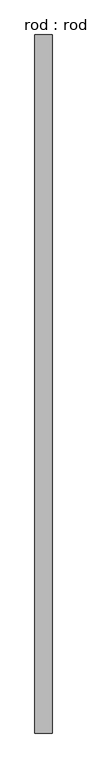
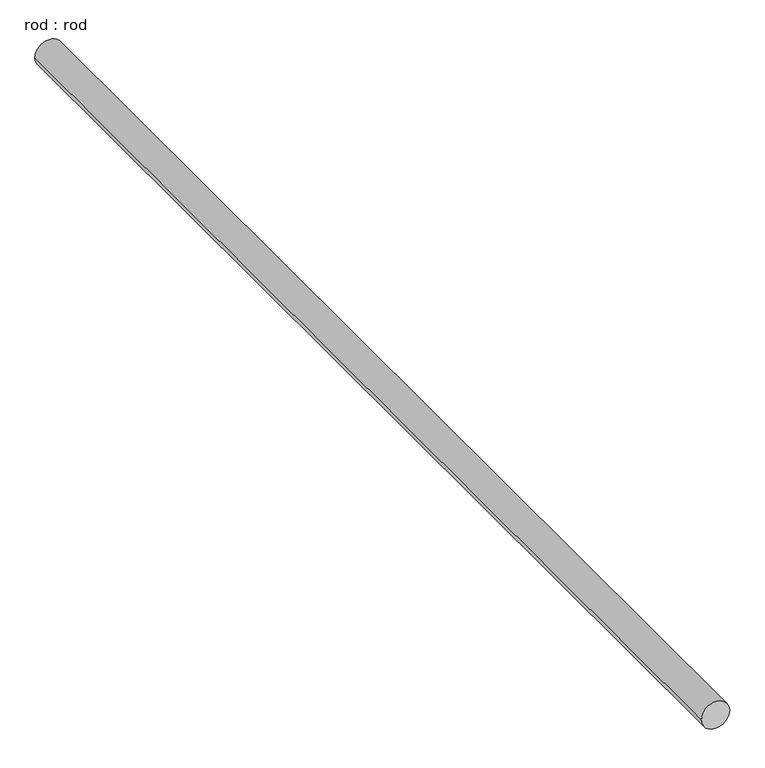
"""IFC4 building model written with IfcOpenShell, lengths in millimetres: proxy geometry, rod : rod."""

from ifc_helpers import new_model, si_unit, point, frame, frame_2d, origin, place, context, project, spatial, circle_curve, trimmed, segment, composite_curve, outline, extrude, source, transform, mapped, element, save


def rod_rod_9af83bd0(model_context):
    return source(origin(), model_context, "Body", "SweptSolid", [
        extrude(outline(composite_curve([segment(trimmed(circle_curve(frame_2d((0.0108462, 0.0)), 200.0), [point((0.0108462, 200.0))], [point((0.0108462, -200.0))], False, "CARTESIAN"), True, "CONTINUOUS"), segment(trimmed(circle_curve(frame_2d((0.0108462, 0.0)), 200.0), [point((0.0108462, -200.0))], [point((0.0108462, 200.0))], False, "CARTESIAN"), True, "CONTINUOUS")], self_intersect=False)), frame((0.0, -4064.193954, 0.0), z_axis=(0.0, 1.0, 0.0), x_axis=(0.0, 0.0, 1.0)), (0.0, 0.0, 1.0), 16313.8451387),
    ])


if __name__ == "__main__":
    model = new_model("IFC4")
    model_context = context("Model", 3, world=origin())
    ifc_project = project(units=[si_unit("LENGTHUNIT", "METRE", prefix="MILLI")], contexts=[model_context])
    site = spatial("IfcSite", under=ifc_project)
    building = spatial("IfcBuilding", under=site)
    placement = place(None, origin())
    rod_rod_shape = rod_rod_9af83bd0(model_context)
    element("IfcBuildingElementProxy", 1, Name="rod : rod", ObjectType="rod : rod", at=placement, inside=building, context=model_context, shape_type="MappedRepresentation", body=[
        mapped(rod_rod_shape, transform((0.0, 0.0, 0.0), x_axis=(1.0, 0.0, 0.0), y_axis=(0.0, 1.0, 0.0), z_axis=(0.0, 0.0, 1.0))),
    ])
    save(model, "model.ifc")

# Revit data of these elements
# Type "rod : rod"
#   Default Elevation = 0
